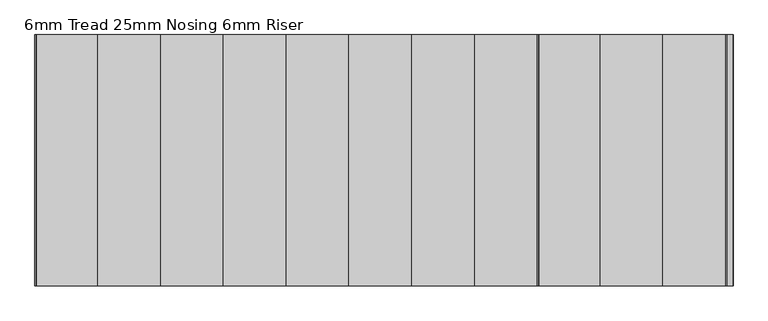
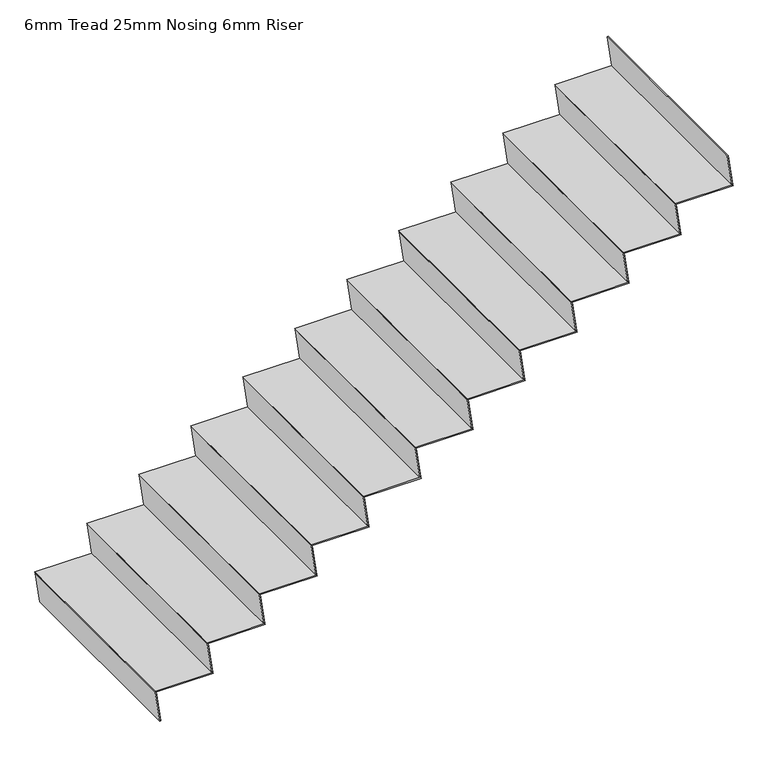
"""IFC4 building model written with IfcOpenShell, lengths in millimetres: stair flight geometry, 6mm Tread 25mm Nosing 6mm Riser."""

import ifcopenshell
import ifcopenshell.guid

model = None  # the IFC model being written
_history = None  # IfcOwnerHistory: only IFC2X3 demands one
_inside = {}  # id of a spatial element -> (the spatial element, [elements in it])
_under = {}  # id of a project, library or spatial element -> (it, [spatial elements below it])
_declared = {}  # id of a project -> (the project, [libraries it declares])
_typed = {}  # id of a type object -> (the type object, [elements of that type])
_made_of = {}  # id of a material, layer set ... -> (it, [elements and type objects made of it])


def new_model(schema):
    """Start an empty IFC model of exactly this schema.

    Asked for "IFC4X3", IfcOpenShell would pick the latest addendum, in which some entities
    have other attributes; the version numbers below select the first issue.
    IFC2X3 requires an IfcOwnerHistory on every rooted entity: one is made here for all.
    """
    global model, _history
    if schema == "IFC4X3":
        model = ifcopenshell.file(schema_version=(4, 3, 0, 0))
    else:
        model = ifcopenshell.file(schema=schema)
    _inside.clear()
    _under.clear()
    _declared.clear()
    _typed.clear()
    _made_of.clear()
    _history = None
    if model.schema == "IFC2X3":
        org = make("IfcOrganization", Name="unknown")
        user = make(
            "IfcPersonAndOrganization",
            ThePerson=make("IfcPerson", FamilyName="unknown"),
            TheOrganization=org,
        )
        app = make(
            "IfcApplication",
            ApplicationDeveloper=org,
            Version="unknown",
            ApplicationFullName="unknown",
            ApplicationIdentifier="unknown",
        )
        _history = make(
            "IfcOwnerHistory",
            OwningUser=user,
            OwningApplication=app,
            ChangeAction="ADDED",
            CreationDate=0,
        )
    return model


def make(cls, **values):
    """One entity of the class cls with the attributes given. An attribute that is None is left unset."""
    return model.create_entity(
        cls, **{name: value for name, value in values.items() if value is not None}
    )


def rooted(cls, **values):
    """An entity with a GlobalId (a new one), such as an element, a storey or a relation."""
    return make(cls, GlobalId=ifcopenshell.guid.new(), OwnerHistory=_history, **values)


def si_unit(unit_type, name, prefix=None):
    """IfcSIUnit, for example si_unit("LENGTHUNIT", "METRE", prefix="MILLI")."""
    return make("IfcSIUnit", UnitType=unit_type, Prefix=prefix, Name=name)


def assignment(units):
    """IfcUnitAssignment: the units of a project."""
    return None if units is None else make("IfcUnitAssignment", Units=units)


def point(xyz):
    """IfcCartesianPoint."""
    return None if xyz is None else make("IfcCartesianPoint", Coordinates=xyz)


def direction(xyz):
    """IfcDirection."""
    return None if xyz is None else make("IfcDirection", DirectionRatios=xyz)


def frame(location, z_axis=None, x_axis=None):
    """IfcAxis2Placement3D, a coordinate frame: its origin and axes. An axis left out is left unset."""
    return make(
        "IfcAxis2Placement3D",
        Location=point(location),
        Axis=direction(z_axis),
        RefDirection=direction(x_axis),
    )


def origin():
    """The frame at (0, 0, 0) with its axes left unset."""
    return frame((0.0, 0.0, 0.0))


def place(relative_to, where):
    """IfcLocalPlacement: puts the frame where relative to a parent placement (None: the world)."""
    return make(
        "IfcLocalPlacement", PlacementRelTo=relative_to, RelativePlacement=where
    )


def context(
    kind, dimensions, precision=None, world=None, true_north=None, identifier=None
):
    """IfcGeometricRepresentationContext, for example the 3D "Model" context."""
    return make(
        "IfcGeometricRepresentationContext",
        ContextIdentifier=identifier,
        ContextType=kind,
        CoordinateSpaceDimension=dimensions,
        Precision=precision,
        WorldCoordinateSystem=world,
        TrueNorth=true_north,
    )


def project(units=None, contexts=None):
    """IfcProject with its units and contexts."""
    return rooted(
        "IfcProject",
        Name="project",
        RepresentationContexts=contexts,
        UnitsInContext=assignment(units),
    )


def spatial(cls, under=None, at=None, **own):
    """A site, building, storey or space (cls), placed at a placement, below another one or the project."""
    s = rooted(cls, ObjectPlacement=at, **own)
    if under is not None:
        _under.setdefault(under.id(), (under, []))[1].append(s)
    return s


def polyline(points):
    """IfcPolyline through the points."""
    return make("IfcPolyline", Points=[point(p) for p in points])


def outline(outer, holes=None, kind="AREA"):
    """IfcArbitraryClosedProfileDef: a profile drawn as a closed curve; with holes, ...WithVoids."""
    if holes is None:
        return make("IfcArbitraryClosedProfileDef", ProfileType=kind, OuterCurve=outer)
    return make(
        "IfcArbitraryProfileDefWithVoids",
        ProfileType=kind,
        OuterCurve=outer,
        InnerCurves=holes,
    )


def extrude(swept, where, along, depth):
    """IfcExtrudedAreaSolid: the profile swept, set in the frame where, extruded along a direction by depth."""
    return make(
        "IfcExtrudedAreaSolid",
        SweptArea=swept,
        Position=where,
        ExtrudedDirection=direction(along),
        Depth=depth,
    )


def shape(context_of_items, identifier, shape_type, items):
    """IfcShapeRepresentation: the items that make up one representation, for example the "Body"."""
    return make(
        "IfcShapeRepresentation",
        ContextOfItems=context_of_items,
        RepresentationIdentifier=identifier,
        RepresentationType=shape_type,
        Items=items,
    )


def source(mapping_origin, context_of_items, identifier, shape_type, items):
    """IfcRepresentationMap: a shape defined once, which mapped items show again and again."""
    return make(
        "IfcRepresentationMap",
        MappingOrigin=mapping_origin,
        MappedRepresentation=shape(context_of_items, identifier, shape_type, items),
    )


def transform(
    local_origin,
    x_axis=None,
    y_axis=None,
    z_axis=None,
    scale=None,
    scale2=None,
    scale3=None,
    uniform=True,
):
    """IfcCartesianTransformationOperator3D, or its non-uniform kind. x_axis, y_axis, z_axis: its Axis1, 2, 3."""
    if uniform:
        return make(
            "IfcCartesianTransformationOperator3D",
            Axis1=direction(x_axis),
            Axis2=direction(y_axis),
            LocalOrigin=point(local_origin),
            Scale=scale,
            Axis3=direction(z_axis),
        )
    return make(
        "IfcCartesianTransformationOperator3DnonUniform",
        Axis1=direction(x_axis),
        Axis2=direction(y_axis),
        LocalOrigin=point(local_origin),
        Scale=scale,
        Axis3=direction(z_axis),
        Scale2=scale2,
        Scale3=scale3,
    )


def mapped(mapping_source, mapping_target):
    """IfcMappedItem: shows the shape of a source again, moved by a transform."""
    return make(
        "IfcMappedItem", MappingSource=mapping_source, MappingTarget=mapping_target
    )


def made_of(thing, what):
    """Note that an element or type object is made of a material, layer set ...; save() writes the relation."""
    if what is not None:
        _made_of.setdefault(what.id(), (what, []))[1].append(thing)
    return thing


def element(
    cls,
    number,
    at=None,
    inside=None,
    cuts=None,
    type_object=None,
    material=None,
    context=None,
    identifier="Body",
    shape_type=None,
    held_by="IfcProductDefinitionShape",
    body=None,
    shapes=None,
    **own,
):
    """One element of the class cls, such as IfcWall. Its Tag is "e" and its number.

    at: its placement. inside: the storey or other place that contains it. cuts: it is an
    opening in that element (IfcRelVoidsElement). A single representation is given by context,
    identifier, shape_type and body (its items); several are given by shapes. held_by: the class
    of the entity that holds the representations. save() writes the other relations.
    """
    e = rooted(cls, Tag="e%d" % number, ObjectPlacement=at, **own)
    if body is not None:
        shapes = [shape(context, identifier, shape_type, body)]
    if shapes is not None:
        e.Representation = make(held_by, Representations=shapes)
    if inside is not None:
        _inside.setdefault(inside.id(), (inside, []))[1].append(e)
    if cuts is not None:
        rooted(
            "IfcRelVoidsElement", RelatingBuildingElement=cuts, RelatedOpeningElement=e
        )
    if type_object is not None:
        _typed.setdefault(type_object.id(), (type_object, []))[1].append(e)
    return made_of(e, material)


def aggregate(whole, parts):
    """IfcRelAggregates: a whole, such as a stair, and the parts it consists of."""
    return rooted("IfcRelAggregates", RelatingObject=whole, RelatedObjects=parts)


def save(model, path):
    """Write the relations noted so far, then the file.

    IfcRelAggregates (storeys below a building ...), IfcRelContainedInSpatialStructure (elements
    in a storey), IfcRelDefinesByType, IfcRelAssociatesMaterial and IfcRelDeclares: one each for
    every whole, place, type object, material and project.
    """
    for whole, parts in _under.values():
        aggregate(whole, parts)
    for where, things in _inside.values():
        rooted(
            "IfcRelContainedInSpatialStructure",
            RelatedElements=things,
            RelatingStructure=where,
        )
    for kind, things in _typed.values():
        rooted("IfcRelDefinesByType", RelatedObjects=things, RelatingType=kind)
    for what, things in _made_of.values():
        rooted("IfcRelAssociatesMaterial", RelatedObjects=things, RelatingMaterial=what)
    for by, libraries in _declared.values():
        rooted("IfcRelDeclares", RelatingContext=by, RelatedDefinitions=libraries)
    model.write(path)


def stair_flight_6mm_tread_25mm_nosing_6mm_riser_2288a60d(model_context):
    return source(origin(), model_context, "Body", "SweptSolid", [
        extrude(outline(polyline([(20176.4705882, 13631.0599092), (20176.4705882, 13325.0), (20170.4705882, 13325.85), (20170.4705882, 13631.9099092), (20176.4705882, 13631.0599092)])), frame((0.0, 10295.4345331, 0.0), z_axis=(0.0, 1.0, 0.0), x_axis=(0.0, 0.0, 1.0)), (0.0, 0.0, 1.0), 1100.0),
        extrude(outline(polyline([(20170.4705882, 13325.85), (20000.0, 13350.0), (20000.0, 13356.0599092), (20170.4705882, 13331.9099092), (20170.4705882, 13325.85)])), frame((0.0, 10295.4345331, 0.0), z_axis=(0.0, 1.0, 0.0), x_axis=(0.0, 0.0, 1.0)), (0.0, 0.0, 1.0), 1100.0),
        extrude(outline(polyline([(20346.9411765, 13600.85), (20176.4705882, 13625.0), (20176.4705882, 13631.0599092), (20346.9411765, 13606.9099092), (20346.9411765, 13600.85)])), frame((0.0, 10295.4345331, 0.0), z_axis=(0.0, 1.0, 0.0), x_axis=(0.0, 0.0, 1.0)), (0.0, 0.0, 1.0), 1100.0),
        extrude(outline(polyline([(20352.9411765, 13906.0599092), (20352.9411765, 13600.0), (20346.9411765, 13600.85), (20346.9411765, 13906.9099092), (20352.9411765, 13906.0599092)])), frame((0.0, 10295.4345331, 0.0), z_axis=(0.0, 1.0, 0.0), x_axis=(0.0, 0.0, 1.0)), (0.0, 0.0, 1.0), 1100.0),
        extrude(outline(polyline([(20523.4117647, 13875.85), (20352.9411765, 13900.0), (20352.9411765, 13906.0599092), (20523.4117647, 13881.9099092), (20523.4117647, 13875.85)])), frame((0.0, 10295.4345331, 0.0), z_axis=(0.0, 1.0, 0.0), x_axis=(0.0, 0.0, 1.0)), (0.0, 0.0, 1.0), 1100.0),
        extrude(outline(polyline([(20529.4117647, 14181.0599092), (20529.4117647, 13875.0), (20523.4117647, 13875.85), (20523.4117647, 14181.9099092), (20529.4117647, 14181.0599092)])), frame((0.0, 10295.4345331, 0.0), z_axis=(0.0, 1.0, 0.0), x_axis=(0.0, 0.0, 1.0)), (0.0, 0.0, 1.0), 1100.0),
        extrude(outline(polyline([(20699.8823529, 14150.85), (20529.4117647, 14175.0), (20529.4117647, 14181.0599092), (20699.8823529, 14156.9099092), (20699.8823529, 14150.85)])), frame((0.0, 10295.4345331, 0.0), z_axis=(0.0, 1.0, 0.0), x_axis=(0.0, 0.0, 1.0)), (0.0, 0.0, 1.0), 1100.0),
        extrude(outline(polyline([(20705.8823529, 14456.0599092), (20705.8823529, 14150.0), (20699.8823529, 14150.85), (20699.8823529, 14456.9099092), (20705.8823529, 14456.0599092)])), frame((0.0, 10295.4345331, 0.0), z_axis=(0.0, 1.0, 0.0), x_axis=(0.0, 0.0, 1.0)), (0.0, 0.0, 1.0), 1100.0),
        extrude(outline(polyline([(20876.3529412, 14425.85), (20705.8823529, 14450.0), (20705.8823529, 14456.0599092), (20876.3529412, 14431.9099092), (20876.3529412, 14425.85)])), frame((0.0, 10295.4345331, 0.0), z_axis=(0.0, 1.0, 0.0), x_axis=(0.0, 0.0, 1.0)), (0.0, 0.0, 1.0), 1100.0),
        extrude(outline(polyline([(20882.3529412, 14731.0599092), (20882.3529412, 14425.0), (20876.3529412, 14425.85), (20876.3529412, 14731.9099092), (20882.3529412, 14731.0599092)])), frame((0.0, 10295.4345331, 0.0), z_axis=(0.0, 1.0, 0.0), x_axis=(0.0, 0.0, 1.0)), (0.0, 0.0, 1.0), 1100.0),
        extrude(outline(polyline([(21052.8235294, 14700.85), (20882.3529412, 14725.0), (20882.3529412, 14731.0599092), (21052.8235294, 14706.9099092), (21052.8235294, 14700.85)])), frame((0.0, 10295.4345331, 0.0), z_axis=(0.0, 1.0, 0.0), x_axis=(0.0, 0.0, 1.0)), (0.0, 0.0, 1.0), 1100.0),
        extrude(outline(polyline([(21058.8235294, 15006.0599092), (21058.8235294, 14700.0), (21052.8235294, 14700.85), (21052.8235294, 15006.9099092), (21058.8235294, 15006.0599092)])), frame((0.0, 10295.4345331, 0.0), z_axis=(0.0, 1.0, 0.0), x_axis=(0.0, 0.0, 1.0)), (0.0, 0.0, 1.0), 1100.0),
        extrude(outline(polyline([(21229.2941176, 14975.85), (21058.8235294, 15000.0), (21058.8235294, 15006.0599092), (21229.2941176, 14981.9099092), (21229.2941176, 14975.85)])), frame((0.0, 10295.4345331, 0.0), z_axis=(0.0, 1.0, 0.0), x_axis=(0.0, 0.0, 1.0)), (0.0, 0.0, 1.0), 1100.0),
        extrude(outline(polyline([(21235.2941176, 15281.0599092), (21235.2941176, 14975.0), (21229.2941176, 14975.85), (21229.2941176, 15281.9099092), (21235.2941176, 15281.0599092)])), frame((0.0, 10295.4345331, 0.0), z_axis=(0.0, 1.0, 0.0), x_axis=(0.0, 0.0, 1.0)), (0.0, 0.0, 1.0), 1100.0),
        extrude(outline(polyline([(21405.7647059, 15250.85), (21235.2941176, 15275.0), (21235.2941176, 15281.0599092), (21405.7647059, 15256.9099092), (21405.7647059, 15250.85)])), frame((0.0, 10295.4345331, 0.0), z_axis=(0.0, 1.0, 0.0), x_axis=(0.0, 0.0, 1.0)), (0.0, 0.0, 1.0), 1100.0),
        extrude(outline(polyline([(21411.7647059, 15556.0599092), (21411.7647059, 15250.0), (21405.7647059, 15250.85), (21405.7647059, 15556.9099092), (21411.7647059, 15556.0599092)])), frame((0.0, 10295.4345331, 0.0), z_axis=(0.0, 1.0, 0.0), x_axis=(0.0, 0.0, 1.0)), (0.0, 0.0, 1.0), 1100.0),
        extrude(outline(polyline([(21582.2352941, 15525.85), (21411.7647059, 15550.0), (21411.7647059, 15556.0599092), (21582.2352941, 15531.9099092), (21582.2352941, 15525.85)])), frame((0.0, 10295.4345331, 0.0), z_axis=(0.0, 1.0, 0.0), x_axis=(0.0, 0.0, 1.0)), (0.0, 0.0, 1.0), 1100.0),
        extrude(outline(polyline([(21588.2352941, 15831.0599092), (21588.2352941, 15525.0), (21582.2352941, 15525.85), (21582.2352941, 15831.9099092), (21588.2352941, 15831.0599092)])), frame((0.0, 10295.4345331, 0.0), z_axis=(0.0, 1.0, 0.0), x_axis=(0.0, 0.0, 1.0)), (0.0, 0.0, 1.0), 1100.0),
        extrude(outline(polyline([(21758.7058824, 15800.85), (21588.2352941, 15825.0), (21588.2352941, 15831.0599092), (21758.7058824, 15806.9099092), (21758.7058824, 15800.85)])), frame((0.0, 10295.4345331, 0.0), z_axis=(0.0, 1.0, 0.0), x_axis=(0.0, 0.0, 1.0)), (0.0, 0.0, 1.0), 1100.0),
        extrude(outline(polyline([(21764.7058824, 16106.0599092), (21764.7058824, 15800.0), (21758.7058824, 15800.85), (21758.7058824, 16106.9099092), (21764.7058824, 16106.0599092)])), frame((0.0, 10295.4345331, 0.0), z_axis=(0.0, 1.0, 0.0), x_axis=(0.0, 0.0, 1.0)), (0.0, 0.0, 1.0), 1100.0),
        extrude(outline(polyline([(21935.1764706, 16075.85), (21764.7058824, 16100.0), (21764.7058824, 16106.0599092), (21935.1764706, 16081.9099092), (21935.1764706, 16075.85)])), frame((0.0, 10295.4345331, 0.0), z_axis=(0.0, 1.0, 0.0), x_axis=(0.0, 0.0, 1.0)), (0.0, 0.0, 1.0), 1100.0),
        extrude(outline(polyline([(22111.6470588, 16350.85), (21941.1764706, 16375.0), (21941.1764706, 16381.0599092), (22111.6470588, 16356.9099092), (22111.6470588, 16350.85)])), frame((0.0, 10295.4345331, 0.0), z_axis=(0.0, 1.0, 0.0), x_axis=(0.0, 0.0, 1.0)), (0.0, 0.0, 1.0), 1100.0),
        extrude(outline(polyline([(21941.1764706, 16381.0599092), (21941.1764706, 16075.0), (21935.1764706, 16075.85), (21935.1764706, 16381.9099092), (21941.1764706, 16381.0599092)])), frame((0.0, 10295.4345331, 0.0), z_axis=(0.0, 1.0, 0.0), x_axis=(0.0, 0.0, 1.0)), (0.0, 0.0, 1.0), 1100.0),
    ])


if __name__ == "__main__":
    model = new_model("IFC4")
    model_context = context("Model", 3, world=origin())
    ifc_project = project(units=[si_unit("LENGTHUNIT", "METRE", prefix="MILLI")], contexts=[model_context])
    site = spatial("IfcSite", under=ifc_project)
    building = spatial("IfcBuilding", under=site)
    placement = place(None, origin())
    stair_flight_6mm_tread_25mm_nosing_6mm_riser_shape = stair_flight_6mm_tread_25mm_nosing_6mm_riser_2288a60d(model_context)
    element("IfcStairFlight", 1, ObjectType="6mm Tread 25mm Nosing 6mm Riser", at=placement, inside=building, context=model_context, shape_type="MappedRepresentation", body=[
        mapped(stair_flight_6mm_tread_25mm_nosing_6mm_riser_shape, transform((0.0, 0.0, 0.0), x_axis=(1.0, 0.0, 0.0), y_axis=(0.0, 1.0, 0.0), z_axis=(0.0, 0.0, 1.0))),
    ])
    save(model, "model.ifc")

# Revit data of these elements
# Element 1 (IfcStairFlight, "6mm Tread 25mm Nosing 6mm Riser")
#   Materials on its faces: "Steel, Paint Finish, Dark Gray"
# Materials
#   "Steel, Paint Finish, Dark Gray": class "Metal", colour RGB 89 89 89, transparency 0, Description = "Steel, paint finish, dark gray, glossy", Cost = 0
